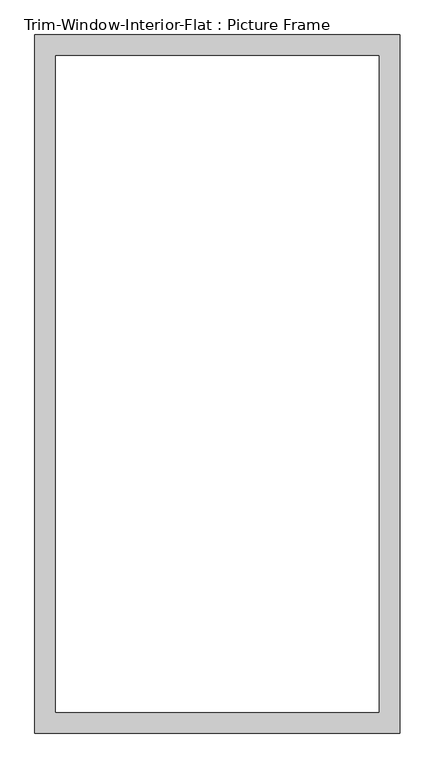
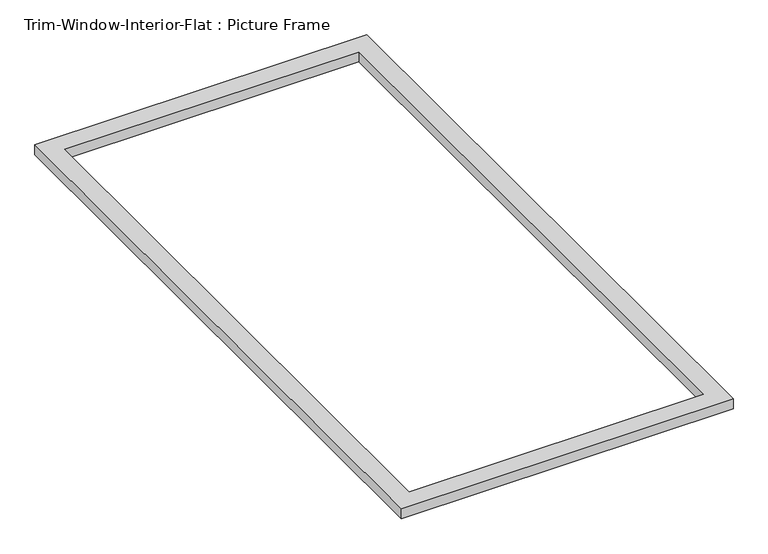
"""IFC4 building model written with IfcOpenShell, lengths in millimetres: proxy geometry, Trim-Window-Interior-Flat : Picture Frame."""

import ifcopenshell
import ifcopenshell.guid

model = None  # the IFC model being written
_history = None  # IfcOwnerHistory: only IFC2X3 demands one
_inside = {}  # id of a spatial element -> (the spatial element, [elements in it])
_under = {}  # id of a project, library or spatial element -> (it, [spatial elements below it])
_declared = {}  # id of a project -> (the project, [libraries it declares])
_typed = {}  # id of a type object -> (the type object, [elements of that type])
_made_of = {}  # id of a material, layer set ... -> (it, [elements and type objects made of it])


def new_model(schema):
    """Start an empty IFC model of exactly this schema.

    Asked for "IFC4X3", IfcOpenShell would pick the latest addendum, in which some entities
    have other attributes; the version numbers below select the first issue.
    IFC2X3 requires an IfcOwnerHistory on every rooted entity: one is made here for all.
    """
    global model, _history
    if schema == "IFC4X3":
        model = ifcopenshell.file(schema_version=(4, 3, 0, 0))
    else:
        model = ifcopenshell.file(schema=schema)
    _inside.clear()
    _under.clear()
    _declared.clear()
    _typed.clear()
    _made_of.clear()
    _history = None
    if model.schema == "IFC2X3":
        org = make("IfcOrganization", Name="unknown")
        user = make(
            "IfcPersonAndOrganization",
            ThePerson=make("IfcPerson", FamilyName="unknown"),
            TheOrganization=org,
        )
        app = make(
            "IfcApplication",
            ApplicationDeveloper=org,
            Version="unknown",
            ApplicationFullName="unknown",
            ApplicationIdentifier="unknown",
        )
        _history = make(
            "IfcOwnerHistory",
            OwningUser=user,
            OwningApplication=app,
            ChangeAction="ADDED",
            CreationDate=0,
        )
    return model


def make(cls, **values):
    """One entity of the class cls with the attributes given. An attribute that is None is left unset."""
    return model.create_entity(
        cls, **{name: value for name, value in values.items() if value is not None}
    )


def rooted(cls, **values):
    """An entity with a GlobalId (a new one), such as an element, a storey or a relation."""
    return make(cls, GlobalId=ifcopenshell.guid.new(), OwnerHistory=_history, **values)


def si_unit(unit_type, name, prefix=None):
    """IfcSIUnit, for example si_unit("LENGTHUNIT", "METRE", prefix="MILLI")."""
    return make("IfcSIUnit", UnitType=unit_type, Prefix=prefix, Name=name)


def assignment(units):
    """IfcUnitAssignment: the units of a project."""
    return None if units is None else make("IfcUnitAssignment", Units=units)


def point(xyz):
    """IfcCartesianPoint."""
    return None if xyz is None else make("IfcCartesianPoint", Coordinates=xyz)


def direction(xyz):
    """IfcDirection."""
    return None if xyz is None else make("IfcDirection", DirectionRatios=xyz)


def frame(location, z_axis=None, x_axis=None):
    """IfcAxis2Placement3D, a coordinate frame: its origin and axes. An axis left out is left unset."""
    return make(
        "IfcAxis2Placement3D",
        Location=point(location),
        Axis=direction(z_axis),
        RefDirection=direction(x_axis),
    )


def origin():
    """The frame at (0, 0, 0) with its axes left unset."""
    return frame((0.0, 0.0, 0.0))


def origin_with_axes():
    """The frame at (0, 0, 0) with the z axis (0, 0, 1) and the x axis (1, 0, 0) written out."""
    return frame((0.0, 0.0, 0.0), z_axis=(0.0, 0.0, 1.0), x_axis=(1.0, 0.0, 0.0))


def place(relative_to, where):
    """IfcLocalPlacement: puts the frame where relative to a parent placement (None: the world)."""
    return make(
        "IfcLocalPlacement", PlacementRelTo=relative_to, RelativePlacement=where
    )


def context(
    kind, dimensions, precision=None, world=None, true_north=None, identifier=None
):
    """IfcGeometricRepresentationContext, for example the 3D "Model" context."""
    return make(
        "IfcGeometricRepresentationContext",
        ContextIdentifier=identifier,
        ContextType=kind,
        CoordinateSpaceDimension=dimensions,
        Precision=precision,
        WorldCoordinateSystem=world,
        TrueNorth=true_north,
    )


def project(units=None, contexts=None):
    """IfcProject with its units and contexts."""
    return rooted(
        "IfcProject",
        Name="project",
        RepresentationContexts=contexts,
        UnitsInContext=assignment(units),
    )


def spatial(cls, under=None, at=None, **own):
    """A site, building, storey or space (cls), placed at a placement, below another one or the project."""
    s = rooted(cls, ObjectPlacement=at, **own)
    if under is not None:
        _under.setdefault(under.id(), (under, []))[1].append(s)
    return s


def polyline(points):
    """IfcPolyline through the points."""
    return make("IfcPolyline", Points=[point(p) for p in points])


def outline(outer, holes=None, kind="AREA"):
    """IfcArbitraryClosedProfileDef: a profile drawn as a closed curve; with holes, ...WithVoids."""
    if holes is None:
        return make("IfcArbitraryClosedProfileDef", ProfileType=kind, OuterCurve=outer)
    return make(
        "IfcArbitraryProfileDefWithVoids",
        ProfileType=kind,
        OuterCurve=outer,
        InnerCurves=holes,
    )


def extrude(swept, where, along, depth):
    """IfcExtrudedAreaSolid: the profile swept, set in the frame where, extruded along a direction by depth."""
    return make(
        "IfcExtrudedAreaSolid",
        SweptArea=swept,
        Position=where,
        ExtrudedDirection=direction(along),
        Depth=depth,
    )


def shape(context_of_items, identifier, shape_type, items):
    """IfcShapeRepresentation: the items that make up one representation, for example the "Body"."""
    return make(
        "IfcShapeRepresentation",
        ContextOfItems=context_of_items,
        RepresentationIdentifier=identifier,
        RepresentationType=shape_type,
        Items=items,
    )


def source(mapping_origin, context_of_items, identifier, shape_type, items):
    """IfcRepresentationMap: a shape defined once, which mapped items show again and again."""
    return make(
        "IfcRepresentationMap",
        MappingOrigin=mapping_origin,
        MappedRepresentation=shape(context_of_items, identifier, shape_type, items),
    )


def transform(
    local_origin,
    x_axis=None,
    y_axis=None,
    z_axis=None,
    scale=None,
    scale2=None,
    scale3=None,
    uniform=True,
):
    """IfcCartesianTransformationOperator3D, or its non-uniform kind. x_axis, y_axis, z_axis: its Axis1, 2, 3."""
    if uniform:
        return make(
            "IfcCartesianTransformationOperator3D",
            Axis1=direction(x_axis),
            Axis2=direction(y_axis),
            LocalOrigin=point(local_origin),
            Scale=scale,
            Axis3=direction(z_axis),
        )
    return make(
        "IfcCartesianTransformationOperator3DnonUniform",
        Axis1=direction(x_axis),
        Axis2=direction(y_axis),
        LocalOrigin=point(local_origin),
        Scale=scale,
        Axis3=direction(z_axis),
        Scale2=scale2,
        Scale3=scale3,
    )


def mapped(mapping_source, mapping_target):
    """IfcMappedItem: shows the shape of a source again, moved by a transform."""
    return make(
        "IfcMappedItem", MappingSource=mapping_source, MappingTarget=mapping_target
    )


def made_of(thing, what):
    """Note that an element or type object is made of a material, layer set ...; save() writes the relation."""
    if what is not None:
        _made_of.setdefault(what.id(), (what, []))[1].append(thing)
    return thing


def element(
    cls,
    number,
    at=None,
    inside=None,
    cuts=None,
    type_object=None,
    material=None,
    context=None,
    identifier="Body",
    shape_type=None,
    held_by="IfcProductDefinitionShape",
    body=None,
    shapes=None,
    **own,
):
    """One element of the class cls, such as IfcWall. Its Tag is "e" and its number.

    at: its placement. inside: the storey or other place that contains it. cuts: it is an
    opening in that element (IfcRelVoidsElement). A single representation is given by context,
    identifier, shape_type and body (its items); several are given by shapes. held_by: the class
    of the entity that holds the representations. save() writes the other relations.
    """
    e = rooted(cls, Tag="e%d" % number, ObjectPlacement=at, **own)
    if body is not None:
        shapes = [shape(context, identifier, shape_type, body)]
    if shapes is not None:
        e.Representation = make(held_by, Representations=shapes)
    if inside is not None:
        _inside.setdefault(inside.id(), (inside, []))[1].append(e)
    if cuts is not None:
        rooted(
            "IfcRelVoidsElement", RelatingBuildingElement=cuts, RelatedOpeningElement=e
        )
    if type_object is not None:
        _typed.setdefault(type_object.id(), (type_object, []))[1].append(e)
    return made_of(e, material)


def aggregate(whole, parts):
    """IfcRelAggregates: a whole, such as a stair, and the parts it consists of."""
    return rooted("IfcRelAggregates", RelatingObject=whole, RelatedObjects=parts)


def save(model, path):
    """Write the relations noted so far, then the file.

    IfcRelAggregates (storeys below a building ...), IfcRelContainedInSpatialStructure (elements
    in a storey), IfcRelDefinesByType, IfcRelAssociatesMaterial and IfcRelDeclares: one each for
    every whole, place, type object, material and project.
    """
    for whole, parts in _under.values():
        aggregate(whole, parts)
    for where, things in _inside.values():
        rooted(
            "IfcRelContainedInSpatialStructure",
            RelatedElements=things,
            RelatingStructure=where,
        )
    for kind, things in _typed.values():
        rooted("IfcRelDefinesByType", RelatedObjects=things, RelatingType=kind)
    for what, things in _made_of.values():
        rooted("IfcRelAssociatesMaterial", RelatedObjects=things, RelatingMaterial=what)
    for by, libraries in _declared.values():
        rooted("IfcRelDeclares", RelatingContext=by, RelatedDefinitions=libraries)
    model.write(path)


def trim_window_interior_flat_picture_frame_a0ba83d5(model_context):
    return source(origin(), model_context, "Body", "SweptSolid", [
        extrude(outline(polyline([(501.65, -44.45), (-501.65, -44.45), (-501.65, 1873.25), (501.65, 1873.25), (501.65, -44.45)]), holes=[polyline([(444.5, 12.7), (444.5, 1816.1), (-444.5, 1816.1), (-444.5, 12.7), (444.5, 12.7)])]), origin_with_axes(), (0.0, 0.0, 1.0), 31.75),
    ])


if __name__ == "__main__":
    model = new_model("IFC4")
    model_context = context("Model", 3, world=origin())
    ifc_project = project(units=[si_unit("LENGTHUNIT", "METRE", prefix="MILLI")], contexts=[model_context])
    site = spatial("IfcSite", under=ifc_project)
    building = spatial("IfcBuilding", under=site)
    placement = place(None, origin())
    trim_window_interior_flat_picture_frame_shape = trim_window_interior_flat_picture_frame_a0ba83d5(model_context)
    element("IfcBuildingElementProxy", 1, Name="Trim-Window-Interior-Flat : Picture Frame", ObjectType="Trim-Window-Interior-Flat : Picture Frame", at=placement, inside=building, context=model_context, shape_type="MappedRepresentation", body=[
        mapped(trim_window_interior_flat_picture_frame_shape, transform((0.0, 0.0, 0.0), x_axis=(1.0, 0.0, 0.0), y_axis=(0.0, 1.0, 0.0), z_axis=(0.0, 0.0, 1.0))),
    ])
    save(model, "model.ifc")

# Revit data of these elements
# Type "Trim-Window-Interior-Flat : Picture Frame"
#   Trim Thickness_Picture Frame = 0' - 1 1/4"
#   Trim Width = 0' - 2 1/4"
#   Trim Thickness_with Sill = 0' - 0 3/4"
#   Sill Thickness = 0' - 1 1/4"
#   Opening Width [instance default] = 2' - 0"
#   Opening Height [instance default] = 3' - 0"
#   Default Elevation = 4' - 0"
#   Sill = no
#   Picture Frame = yes
#   Trim Material [instance default] = none
# Element 1 (IfcBuildingElementProxy, "Trim-Window-Interior-Flat : Picture Frame")
#   Opening Width = 3' - 0"
#   Opening Height = 6' - 0"
#   Trim Material = Wood - Stained
#   Materials on its faces: "Wood - Stained"
# Materials
#   "Wood - Stained": class "Wood", colour RGB 224 178 126, transparency 0, Cost = 0
